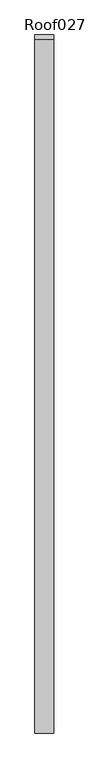
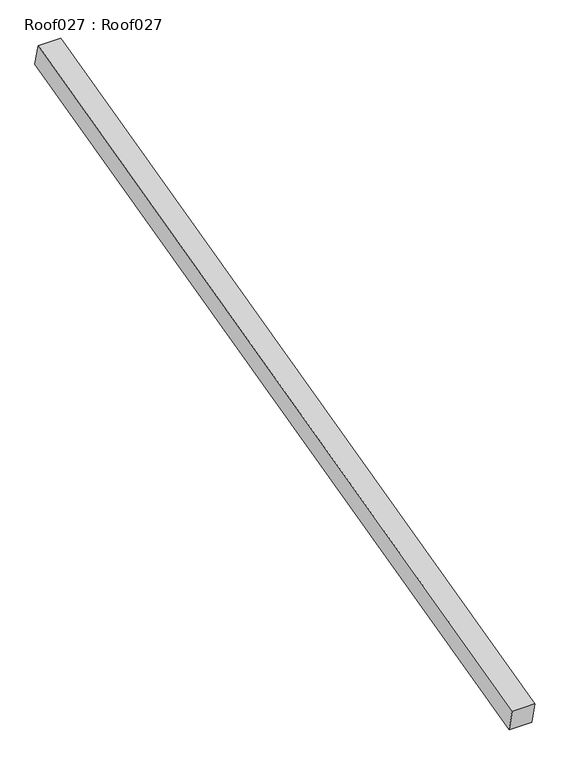
"""IFC4 building model written with IfcOpenShell, lengths in millimetres: proxy geometry, Roof027 : Roof027."""

from ifc_helpers import new_model, si_unit, frame, origin, place, context, project, spatial, polyline, outline, extrude, source, transform, mapped, element, save


def roof027_roof027_e7c44717(model_context):
    return source(origin(), model_context, "Body", "SweptSolid", [
        extrude(outline(polyline([(-5247.7454625, 42918.7637785), (-3387.8525218, 43383.7351117), (-3374.6403653, 43330.8858071), (-5234.533306, 42865.9144738), (-5247.7454625, 42918.7637785)])), frame((12580.6064453, 0.0, 0.0), z_axis=(1.0, 0.0, 0.0), x_axis=(0.0, 1.0, 0.0)), (0.0, 0.0, 1.0), 50.8),
    ])


if __name__ == "__main__":
    model = new_model("IFC4")
    model_context = context("Model", 3, world=origin())
    ifc_project = project(units=[si_unit("LENGTHUNIT", "METRE", prefix="MILLI")], contexts=[model_context])
    site = spatial("IfcSite", under=ifc_project)
    building = spatial("IfcBuilding", under=site)
    placement = place(None, origin())
    roof027_roof027_shape = roof027_roof027_e7c44717(model_context)
    element("IfcBuildingElementProxy", 1, Name="Roof027 : Roof027", ObjectType="Roof027 : Roof027", at=placement, inside=building, context=model_context, shape_type="MappedRepresentation", body=[
        mapped(roof027_roof027_shape, transform((0.0, 0.0, 0.0), x_axis=(1.0, 0.0, 0.0), y_axis=(0.0, 1.0, 0.0), z_axis=(0.0, 0.0, 1.0))),
    ])
    save(model, "model.ifc")

# Revit data of these elements
# Type "Roof027 : Roof027"
#   NameOverride = "Roof027"
# Element 1 (IfcBuildingElementProxy, "Roof027 : Roof027")
#   Materials on its faces: "STANDING SEAM METAL ROOF"
# Materials
#   "STANDING SEAM METAL ROOF": class "Unassigned", colour RGB 128 128 128, transparency 0
